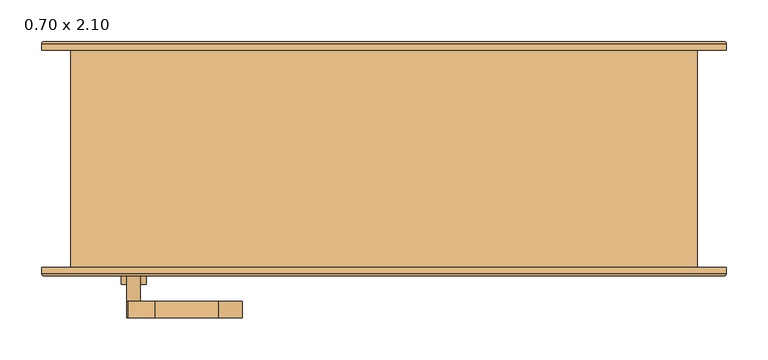
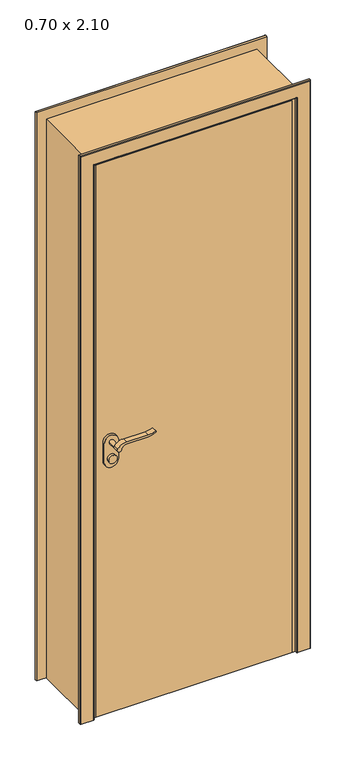
"""IFC4 building model written with IfcOpenShell, lengths in millimetres: door geometry, .CC_ND 300_PORTA SIMPLES DE ABRIR_COM EXTENSÃO : 0.70 x 2.10."""

import ifcopenshell
import ifcopenshell.guid

model = None  # the IFC model being written
_history = None  # IfcOwnerHistory: only IFC2X3 demands one
_inside = {}  # id of a spatial element -> (the spatial element, [elements in it])
_under = {}  # id of a project, library or spatial element -> (it, [spatial elements below it])
_declared = {}  # id of a project -> (the project, [libraries it declares])
_typed = {}  # id of a type object -> (the type object, [elements of that type])
_made_of = {}  # id of a material, layer set ... -> (it, [elements and type objects made of it])


def new_model(schema):
    """Start an empty IFC model of exactly this schema.

    Asked for "IFC4X3", IfcOpenShell would pick the latest addendum, in which some entities
    have other attributes; the version numbers below select the first issue.
    IFC2X3 requires an IfcOwnerHistory on every rooted entity: one is made here for all.
    """
    global model, _history
    if schema == "IFC4X3":
        model = ifcopenshell.file(schema_version=(4, 3, 0, 0))
    else:
        model = ifcopenshell.file(schema=schema)
    _inside.clear()
    _under.clear()
    _declared.clear()
    _typed.clear()
    _made_of.clear()
    _history = None
    if model.schema == "IFC2X3":
        org = make("IfcOrganization", Name="unknown")
        user = make(
            "IfcPersonAndOrganization",
            ThePerson=make("IfcPerson", FamilyName="unknown"),
            TheOrganization=org,
        )
        app = make(
            "IfcApplication",
            ApplicationDeveloper=org,
            Version="unknown",
            ApplicationFullName="unknown",
            ApplicationIdentifier="unknown",
        )
        _history = make(
            "IfcOwnerHistory",
            OwningUser=user,
            OwningApplication=app,
            ChangeAction="ADDED",
            CreationDate=0,
        )
    return model


def make(cls, **values):
    """One entity of the class cls with the attributes given. An attribute that is None is left unset."""
    return model.create_entity(
        cls, **{name: value for name, value in values.items() if value is not None}
    )


def rooted(cls, **values):
    """An entity with a GlobalId (a new one), such as an element, a storey or a relation."""
    return make(cls, GlobalId=ifcopenshell.guid.new(), OwnerHistory=_history, **values)


def si_unit(unit_type, name, prefix=None):
    """IfcSIUnit, for example si_unit("LENGTHUNIT", "METRE", prefix="MILLI")."""
    return make("IfcSIUnit", UnitType=unit_type, Prefix=prefix, Name=name)


def assignment(units):
    """IfcUnitAssignment: the units of a project."""
    return None if units is None else make("IfcUnitAssignment", Units=units)


def point(xyz):
    """IfcCartesianPoint."""
    return None if xyz is None else make("IfcCartesianPoint", Coordinates=xyz)


def direction(xyz):
    """IfcDirection."""
    return None if xyz is None else make("IfcDirection", DirectionRatios=xyz)


def frame(location, z_axis=None, x_axis=None):
    """IfcAxis2Placement3D, a coordinate frame: its origin and axes. An axis left out is left unset."""
    return make(
        "IfcAxis2Placement3D",
        Location=point(location),
        Axis=direction(z_axis),
        RefDirection=direction(x_axis),
    )


def frame_2d(location, x_axis=None):
    """IfcAxis2Placement2D, a coordinate frame in the plane: its origin and x axis."""
    return make(
        "IfcAxis2Placement2D", Location=point(location), RefDirection=direction(x_axis)
    )


def origin():
    """The frame at (0, 0, 0) with its axes left unset."""
    return frame((0.0, 0.0, 0.0))


def origin_with_axes():
    """The frame at (0, 0, 0) with the z axis (0, 0, 1) and the x axis (1, 0, 0) written out."""
    return frame((0.0, 0.0, 0.0), z_axis=(0.0, 0.0, 1.0), x_axis=(1.0, 0.0, 0.0))


def place(relative_to, where):
    """IfcLocalPlacement: puts the frame where relative to a parent placement (None: the world)."""
    return make(
        "IfcLocalPlacement", PlacementRelTo=relative_to, RelativePlacement=where
    )


def context(
    kind, dimensions, precision=None, world=None, true_north=None, identifier=None
):
    """IfcGeometricRepresentationContext, for example the 3D "Model" context."""
    return make(
        "IfcGeometricRepresentationContext",
        ContextIdentifier=identifier,
        ContextType=kind,
        CoordinateSpaceDimension=dimensions,
        Precision=precision,
        WorldCoordinateSystem=world,
        TrueNorth=true_north,
    )


def project(units=None, contexts=None):
    """IfcProject with its units and contexts."""
    return rooted(
        "IfcProject",
        Name="project",
        RepresentationContexts=contexts,
        UnitsInContext=assignment(units),
    )


def spatial(cls, under=None, at=None, **own):
    """A site, building, storey or space (cls), placed at a placement, below another one or the project."""
    s = rooted(cls, ObjectPlacement=at, **own)
    if under is not None:
        _under.setdefault(under.id(), (under, []))[1].append(s)
    return s


def polyline(points):
    """IfcPolyline through the points."""
    return make("IfcPolyline", Points=[point(p) for p in points])


def circle_curve(where, radius):
    """IfcCircle in the frame where."""
    return make("IfcCircle", Position=where, Radius=radius)


def ellipse_curve(where, semi_axis1, semi_axis2):
    """IfcEllipse in the frame where."""
    return make(
        "IfcEllipse", Position=where, SemiAxis1=semi_axis1, SemiAxis2=semi_axis2
    )


def trimmed(basis, trim1, trim2, sense, master):
    """IfcTrimmedCurve: the piece of a basis curve between two trims."""
    return make(
        "IfcTrimmedCurve",
        BasisCurve=basis,
        Trim1=trim1,
        Trim2=trim2,
        SenseAgreement=sense,
        MasterRepresentation=master,
    )


def segment(curve, same_sense, transition):
    """IfcCompositeCurveSegment."""
    return make(
        "IfcCompositeCurveSegment",
        Transition=transition,
        SameSense=same_sense,
        ParentCurve=curve,
    )


def composite_curve(segments, self_intersect=None):
    """IfcCompositeCurve: segments joined end to end."""
    return make("IfcCompositeCurve", Segments=segments, SelfIntersect=self_intersect)


def outline(outer, holes=None, kind="AREA"):
    """IfcArbitraryClosedProfileDef: a profile drawn as a closed curve; with holes, ...WithVoids."""
    if holes is None:
        return make("IfcArbitraryClosedProfileDef", ProfileType=kind, OuterCurve=outer)
    return make(
        "IfcArbitraryProfileDefWithVoids",
        ProfileType=kind,
        OuterCurve=outer,
        InnerCurves=holes,
    )


def extrude(swept, where, along, depth):
    """IfcExtrudedAreaSolid: the profile swept, set in the frame where, extruded along a direction by depth."""
    return make(
        "IfcExtrudedAreaSolid",
        SweptArea=swept,
        Position=where,
        ExtrudedDirection=direction(along),
        Depth=depth,
    )


def faces_of(points, faces, orient=None, outer=None):
    """IfcFace entities. A face is a list of loops; a loop is a list of indices into points, from 0.

    orient and outer hold one flag for each loop. By default every Orientation is true, the
    first loop of a face is its IfcFaceOuterBound and the others are IfcFaceBound.
    """
    made = []
    for i, loops in enumerate(faces):
        bounds = []
        for j, loop in enumerate(loops):
            is_outer = j == 0 if outer is None else outer[i][j]
            bounds.append(
                make(
                    "IfcFaceOuterBound" if is_outer else "IfcFaceBound",
                    Bound=make("IfcPolyLoop", Polygon=[points[k] for k in loop]),
                    Orientation=True if orient is None else orient[i][j],
                )
            )
        made.append(make("IfcFace", Bounds=bounds))
    return made


def faceted_brep(points, faces, orient=None, outer=None, voids=None):
    """IfcFacetedBrep: a solid bounded by flat faces; with voids (closed shells), ...WithVoids."""
    shared = [point(p) for p in points]
    hull = make("IfcClosedShell", CfsFaces=faces_of(shared, faces, orient, outer))
    if voids is None:
        return make("IfcFacetedBrep", Outer=hull)
    return make(
        "IfcFacetedBrepWithVoids",
        Outer=hull,
        Voids=[
            make(cls, CfsFaces=faces_of(shared, fs, o, b)) for cls, fs, o, b in voids
        ],
    )


def shape(context_of_items, identifier, shape_type, items):
    """IfcShapeRepresentation: the items that make up one representation, for example the "Body"."""
    return make(
        "IfcShapeRepresentation",
        ContextOfItems=context_of_items,
        RepresentationIdentifier=identifier,
        RepresentationType=shape_type,
        Items=items,
    )


def source(mapping_origin, context_of_items, identifier, shape_type, items):
    """IfcRepresentationMap: a shape defined once, which mapped items show again and again."""
    return make(
        "IfcRepresentationMap",
        MappingOrigin=mapping_origin,
        MappedRepresentation=shape(context_of_items, identifier, shape_type, items),
    )


def transform(
    local_origin,
    x_axis=None,
    y_axis=None,
    z_axis=None,
    scale=None,
    scale2=None,
    scale3=None,
    uniform=True,
):
    """IfcCartesianTransformationOperator3D, or its non-uniform kind. x_axis, y_axis, z_axis: its Axis1, 2, 3."""
    if uniform:
        return make(
            "IfcCartesianTransformationOperator3D",
            Axis1=direction(x_axis),
            Axis2=direction(y_axis),
            LocalOrigin=point(local_origin),
            Scale=scale,
            Axis3=direction(z_axis),
        )
    return make(
        "IfcCartesianTransformationOperator3DnonUniform",
        Axis1=direction(x_axis),
        Axis2=direction(y_axis),
        LocalOrigin=point(local_origin),
        Scale=scale,
        Axis3=direction(z_axis),
        Scale2=scale2,
        Scale3=scale3,
    )


def mapped(mapping_source, mapping_target):
    """IfcMappedItem: shows the shape of a source again, moved by a transform."""
    return make(
        "IfcMappedItem", MappingSource=mapping_source, MappingTarget=mapping_target
    )


def made_of(thing, what):
    """Note that an element or type object is made of a material, layer set ...; save() writes the relation."""
    if what is not None:
        _made_of.setdefault(what.id(), (what, []))[1].append(thing)
    return thing


def element(
    cls,
    number,
    at=None,
    inside=None,
    cuts=None,
    type_object=None,
    material=None,
    context=None,
    identifier="Body",
    shape_type=None,
    held_by="IfcProductDefinitionShape",
    body=None,
    shapes=None,
    **own,
):
    """One element of the class cls, such as IfcWall. Its Tag is "e" and its number.

    at: its placement. inside: the storey or other place that contains it. cuts: it is an
    opening in that element (IfcRelVoidsElement). A single representation is given by context,
    identifier, shape_type and body (its items); several are given by shapes. held_by: the class
    of the entity that holds the representations. save() writes the other relations.
    """
    e = rooted(cls, Tag="e%d" % number, ObjectPlacement=at, **own)
    if body is not None:
        shapes = [shape(context, identifier, shape_type, body)]
    if shapes is not None:
        e.Representation = make(held_by, Representations=shapes)
    if inside is not None:
        _inside.setdefault(inside.id(), (inside, []))[1].append(e)
    if cuts is not None:
        rooted(
            "IfcRelVoidsElement", RelatingBuildingElement=cuts, RelatedOpeningElement=e
        )
    if type_object is not None:
        _typed.setdefault(type_object.id(), (type_object, []))[1].append(e)
    return made_of(e, material)


def aggregate(whole, parts):
    """IfcRelAggregates: a whole, such as a stair, and the parts it consists of."""
    return rooted("IfcRelAggregates", RelatingObject=whole, RelatedObjects=parts)


def save(model, path):
    """Write the relations noted so far, then the file.

    IfcRelAggregates (storeys below a building ...), IfcRelContainedInSpatialStructure (elements
    in a storey), IfcRelDefinesByType, IfcRelAssociatesMaterial and IfcRelDeclares: one each for
    every whole, place, type object, material and project.
    """
    for whole, parts in _under.values():
        aggregate(whole, parts)
    for where, things in _inside.values():
        rooted(
            "IfcRelContainedInSpatialStructure",
            RelatedElements=things,
            RelatingStructure=where,
        )
    for kind, things in _typed.values():
        rooted("IfcRelDefinesByType", RelatedObjects=things, RelatingType=kind)
    for what, things in _made_of.values():
        rooted("IfcRelAssociatesMaterial", RelatedObjects=things, RelatingMaterial=what)
    for by, libraries in _declared.values():
        rooted("IfcRelDeclares", RelatingContext=by, RelatedDefinitions=libraries)
    model.write(path)


def plane_surface(at):
    """IfcPlane: the flat surface through the origin of the frame at, square to its z axis."""
    return make("IfcPlane", Position=at)


def cylinder_surface(at, radius):
    """IfcCylindricalSurface: all points at the distance radius from the z axis of the frame at."""
    return make("IfcCylindricalSurface", Position=at, Radius=radius)


def advanced_brep(points, edges, surfaces, faces):
    """IfcAdvancedBrep: a solid bounded by faces that lie on surfaces and meet in shared edges.

    An edge is (start, end): straight between two places in points (the first is 0);
    or (start, end, curve); or (start, end, curve, False) where it runs against its curve.
    A face is (place in surfaces, loops), or (place, loops, False) where it looks against
    its surface's normal. A loop lists edges by number (the first is 1), with a minus sign
    where the edge is run from its end to its start. The first loop is the outer one.
    """
    corners = [point(p) for p in points]
    vertices = [make("IfcVertexPoint", VertexGeometry=c) for c in corners]
    made = []
    for start, end, *more in edges:
        made.append(
            make(
                "IfcEdgeCurve",
                EdgeStart=vertices[start],
                EdgeEnd=vertices[end],
                EdgeGeometry=more[0] if more else make("IfcPolyline", Points=[corners[start], corners[end]]),
                SameSense=more[1] if len(more) > 1 else True,
            )
        )
    hull = []
    for where, loops, *sense in faces:
        bounds = []
        for j, loop in enumerate(loops):
            ring = [make("IfcOrientedEdge", EdgeElement=made[abs(k) - 1], Orientation=k > 0) for k in loop]
            bounds.append(
                make(
                    "IfcFaceOuterBound" if j == 0 else "IfcFaceBound",
                    Bound=make("IfcEdgeLoop", EdgeList=ring),
                    Orientation=True,
                )
            )
        hull.append(make("IfcAdvancedFace", Bounds=bounds, FaceSurface=surfaces[where], SameSense=sense[0] if sense else True))
    return make("IfcAdvancedBrep", Outer=make("IfcClosedShell", CfsFaces=hull))


def door_0_70_x_2_10_365ff999(model_context):
    return source(origin(), model_context, "Body", "SolidModel", [
        extrude(outline(composite_curve([segment(trimmed(circle_curve(frame_2d((964.5, -300.0)), 15.0), [point((964.5, -285.0))], [point((964.5, -315.0))], False, "CARTESIAN"), True, "CONTINUOUS"), segment(trimmed(circle_curve(frame_2d((964.5, -300.0)), 15.0), [point((964.5, -315.0))], [point((964.5, -285.0))], False, "CARTESIAN"), True, "CONTINUOUS")], self_intersect=False)), frame((0.0, -163.0, 0.0), z_axis=(0.0, 1.0, 0.0), x_axis=(0.0, 0.0, 1.0)), (0.0, 0.0, 1.0), 10.0),
        extrude(outline(composite_curve([segment(trimmed(circle_curve(frame_2d((964.5, -300.0)), 15.0), [point((964.5, -285.0))], [point((964.5, -315.0))], False, "CARTESIAN"), True, "CONTINUOUS"), segment(trimmed(circle_curve(frame_2d((964.5, -300.0)), 15.0), [point((964.5, -315.0))], [point((964.5, -285.0))], False, "CARTESIAN"), True, "CONTINUOUS")], self_intersect=False)), frame((0.0, -103.0, 0.0), z_axis=(0.0, 1.0, 0.0), x_axis=(0.0, 0.0, 1.0)), (0.0, 0.0, 1.0), 10.0),
        extrude(outline(composite_curve([segment(trimmed(circle_curve(frame_2d((1024.5, -300.0)), 8.0), [point((1029.1523287, -306.5081363))], [point((1024.5, -292.0))], False, "CARTESIAN"), True, "CONTINUOUS"), segment(trimmed(circle_curve(frame_2d((1019.3738613, -274.6138099)), 18.1261387), [point((1024.5, -292.0))], [point((1037.5, -274.6138099))], True, "CARTESIAN"), True, "CONTINUOUS"), segment(polyline([(1037.5, -274.6138099), (1037.5, -198.3564091)]), True, "CONTINUOUS"), segment(trimmed(circle_curve(frame_2d((1096.7709207, -201.9396612)), 59.3791355), [point((1037.5, -198.3564091))], [point((1046.7135558, -170.0))], False, "CARTESIAN"), True, "CONTINUOUS"), segment(polyline([(1046.7135558, -170.0), (1049.5, -170.0)]), True, "CONTINUOUS"), segment(trimmed(circle_curve(frame_2d((1127.7850638, -198.4227909)), 83.2850902), [point((1049.5, -170.0))], [point((1044.5, -198.3564091))], True, "CARTESIAN"), True, "CONTINUOUS"), segment(polyline([(1044.5, -198.3564091), (1044.5, -274.6325667)]), True, "CONTINUOUS"), segment(trimmed(circle_curve(frame_2d((1007.2555521, -276.3324871)), 37.2832219), [point((1044.5, -274.6325667))], [point((1029.1523287, -306.5081363))], False, "CARTESIAN"), True, "CONTINUOUS")], self_intersect=False)), frame((0.0, -203.0, 0.0), z_axis=(0.0, 1.0, 0.0), x_axis=(0.0, 0.0, 1.0)), (0.0, 0.0, 1.0), 20.0),
        extrude(outline(composite_curve([segment(trimmed(circle_curve(frame_2d((1019.3738682, -274.6138122)), 18.1261318), [point((1024.4999903, -292.0))], [point((1037.5, -274.6138122))], True, "CARTESIAN"), True, "CONTINUOUS"), segment(polyline([(1037.5, -274.6138122), (1037.5, -198.3564091)]), True, "CONTINUOUS"), segment(trimmed(circle_curve(frame_2d((1096.7709207, -201.9396612)), 59.3791355), [point((1037.5, -198.3564091))], [point((1046.7135558, -170.0))], False, "CARTESIAN"), True, "CONTINUOUS"), segment(polyline([(1046.7135558, -170.0), (1049.5, -170.0)]), True, "CONTINUOUS"), segment(trimmed(circle_curve(frame_2d((1127.7850638, -198.4227909)), 83.2850902), [point((1049.5, -170.0))], [point((1044.5, -198.3564091))], True, "CARTESIAN"), True, "CONTINUOUS"), segment(polyline([(1044.5, -198.3564091), (1044.5, -274.6325667)]), True, "CONTINUOUS"), segment(trimmed(circle_curve(frame_2d((1007.2555521, -276.3324871)), 37.2832219), [point((1044.5, -274.6325667))], [point((1029.1523287, -306.5081363))], False, "CARTESIAN"), True, "CONTINUOUS"), segment(trimmed(circle_curve(frame_2d((1024.5, -300.0)), 8.0), [point((1029.1523287, -306.5081363))], [point((1024.4999903, -292.0))], False, "CARTESIAN"), True, "CONTINUOUS")], self_intersect=False)), frame((0.0, -73.0, 0.0), z_axis=(0.0, 1.0, 0.0), x_axis=(0.0, 0.0, 1.0)), (0.0, 0.0, 1.0), 20.0),
        extrude(outline(composite_curve([segment(trimmed(circle_curve(frame_2d((1024.5, -300.0)), 8.0), [point((1024.5, -292.0))], [point((1024.5, -308.0))], False, "CARTESIAN"), True, "CONTINUOUS"), segment(trimmed(circle_curve(frame_2d((1024.5, -300.0)), 8.0), [point((1024.5, -308.0))], [point((1024.5, -292.0))], False, "CARTESIAN"), True, "CONTINUOUS")], self_intersect=False)), frame((0.0, -183.0, 0.0), z_axis=(0.0, 1.0, 0.0), x_axis=(0.0, 0.0, 1.0)), (0.0, 0.0, 1.0), 30.0),
        extrude(outline(composite_curve([segment(trimmed(circle_curve(frame_2d((1024.5, -300.0)), 8.0), [point((1024.5, -292.0))], [point((1024.5, -308.0))], False, "CARTESIAN"), True, "CONTINUOUS"), segment(trimmed(circle_curve(frame_2d((1024.5, -300.0)), 8.0), [point((1024.5, -308.0))], [point((1024.5, -292.0))], False, "CARTESIAN"), True, "CONTINUOUS")], self_intersect=False)), frame((0.0, -103.0, 0.0), z_axis=(0.0, 1.0, 0.0), x_axis=(0.0, 0.0, 1.0)), (0.0, 0.0, 1.0), 30.0),
        extrude(outline(composite_curve([segment(trimmed(circle_curve(frame_2d((954.5, -300.0)), 25.0), [point((954.5, -325.0))], [point((954.5, -275.0))], False, "CARTESIAN"), True, "CONTINUOUS"), segment(polyline([(954.5, -275.0), (1024.5, -275.0)]), True, "CONTINUOUS"), segment(trimmed(circle_curve(frame_2d((1024.5, -300.0)), 25.0), [point((1024.5, -275.0))], [point((1024.5, -325.0))], False, "CARTESIAN"), True, "CONTINUOUS"), segment(polyline([(1024.5, -325.0), (954.5, -325.0)]), True, "CONTINUOUS")], self_intersect=False)), frame((0.0, -153.0, 0.0), z_axis=(0.0, 1.0, 0.0), x_axis=(0.0, 0.0, 1.0)), (0.0, 0.0, 1.0), 10.0),
        extrude(outline(composite_curve([segment(trimmed(circle_curve(frame_2d((954.5, -300.0)), 25.0), [point((954.5, -325.0))], [point((954.5, -275.0))], False, "CARTESIAN"), True, "CONTINUOUS"), segment(polyline([(954.5, -275.0), (1024.5, -275.0)]), True, "CONTINUOUS"), segment(trimmed(circle_curve(frame_2d((1024.5, -300.0)), 25.0), [point((1024.5, -275.0))], [point((1024.5, -325.0))], False, "CARTESIAN"), True, "CONTINUOUS"), segment(polyline([(1024.5, -325.0), (954.5, -325.0)]), True, "CONTINUOUS")], self_intersect=False)), frame((0.0, -113.0, 0.0), z_axis=(0.0, 1.0, 0.0), x_axis=(0.0, 0.0, 1.0)), (0.0, 0.0, 1.0), 10.0),
        advanced_brep(
        [(-410.0, -143.0, 0.0), (-360.0, -143.0, 0.0), (-360.0, -150.0, 0.0), (-363.0, -153.0, 0.0), (-407.0, -153.0, 0.0), (-410.0, -150.0, 0.0), (-410.0, -143.0, 2135.0), (410.0, -143.0, 2135.0), (410.0, -143.0, 0.0), (360.0, -143.0, 0.0), (360.0, -143.0, 2085.0), (-360.0, -143.0, 2085.0), (-360.0, -150.0, 2085.0), (-363.0, -153.0, 2088.0), (363.0, -153.0, 2088.0), (363.0, -153.0, 0.0), (407.0, -153.0, 0.0), (407.0, -153.0, 2132.0), (-407.0, -153.0, 2132.0), (-410.0, -150.0, 2135.0), (410.0, -150.0, 2135.0), (410.0, -150.0, 0.0), (360.0, -150.0, 0.0), (360.0, -150.0, 2085.0)],
        [
            (0, 1),
            (1, 2),
            (2, 3, circle_curve(frame((-363.0, -150.0, 0.0), z_axis=(0.0, 0.0, -1.0), x_axis=(1.0, 0.0, 0.0)), 3.0)),
            (3, 4),
            (4, 5, circle_curve(frame((-407.0, -150.0, 0.0), z_axis=(0.0, 0.0, -1.0), x_axis=(1.0, 0.0, 0.0)), 3.0)),
            (5, 0),
            (0, 6),
            (6, 7),
            (7, 8),
            (8, 9),
            (9, 10),
            (10, 11),
            (11, 1),
            (11, 12),
            (12, 2),
            (12, 13, ellipse_curve(frame((-363.0, -150.0, 2088.0), z_axis=(-0.7071067811865475, 0.0, -0.7071067811865475), x_axis=(0.7071067811865474, 0.0, -0.7071067811865476)), 4.2426407, 3.0)),
            (13, 3),
            (13, 14),
            (14, 15),
            (15, 16),
            (16, 17),
            (17, 18),
            (18, 4),
            (18, 19, ellipse_curve(frame((-407.0, -150.0, 2132.0), z_axis=(-0.7071067811865475, 0.0, -0.7071067811865475), x_axis=(0.7071067811865474, 0.0, -0.7071067811865476)), 4.2426407, 3.0)),
            (19, 5),
            (19, 6),
            (7, 20),
            (20, 21),
            (21, 8),
            (21, 16, circle_curve(frame((407.0, -150.0, 0.0), z_axis=(0.0, 0.0, -1.0), x_axis=(-1.0, 0.0, 0.0)), 3.0)),
            (15, 22, circle_curve(frame((363.0, -150.0, 0.0), z_axis=(0.0, 0.0, -1.0), x_axis=(-1.0, 0.0, 0.0)), 3.0)),
            (22, 9),
            (23, 10),
            (22, 23),
            (14, 23, ellipse_curve(frame((363.0, -150.0, 2088.0), z_axis=(0.7071067811865475, 0.0, -0.7071067811865475), x_axis=(0.7071067811865474, 0.0, 0.7071067811865476)), 4.2426407, 3.0)),
            (20, 17, ellipse_curve(frame((407.0, -150.0, 2132.0), z_axis=(0.7071067811865475, 0.0, -0.7071067811865475), x_axis=(0.7071067811865474, 0.0, 0.7071067811865476)), 4.2426407, 3.0)),
            (23, 12),
            (19, 20),
        ],
        [
            plane_surface(frame((-360.0, -143.0, 0.0), z_axis=(0.0, 0.0, -1.0), x_axis=(0.0, 1.0, 0.0))),
            plane_surface(frame((-410.0, -143.0, 0.0), z_axis=(0.0, 1.0, 0.0), x_axis=(0.0, 0.0, 1.0))),
            plane_surface(frame((-360.0, -143.0, 0.0), z_axis=(1.0, 0.0, 0.0), x_axis=(0.0, 0.0, 1.0))),
            cylinder_surface(frame((-363.0, -150.0, 0.0), z_axis=(0.0, 0.0, -1.0), x_axis=(1.0, 0.0, 0.0)), 3.0),
            plane_surface(frame((-363.0, -153.0, 0.0), z_axis=(0.0, -1.0, 0.0), x_axis=(0.0, 0.0, 1.0))),
            cylinder_surface(frame((-407.0, -150.0, 0.0), z_axis=(0.0, 0.0, -1.0), x_axis=(1.0, 0.0, 0.0)), 3.0),
            plane_surface(frame((-410.0, -150.0, 0.0), z_axis=(-1.0, 0.0, 0.0), x_axis=(0.0, 0.0, 1.0))),
            plane_surface(frame((410.0, -150.0, 2135.0), z_axis=(1.0, 0.0, 0.0), x_axis=(0.0, 0.0, -1.0))),
            plane_surface(frame((360.0, -143.0, 0.0), z_axis=(0.0, 0.0, -1.0), x_axis=(0.0, 1.0, 0.0))),
            plane_surface(frame((360.0, -143.0, 2085.0), z_axis=(-1.0, 0.0, 0.0), x_axis=(0.0, 0.0, -1.0))),
            cylinder_surface(frame((363.0, -150.0, 2085.0), z_axis=(0.0, 0.0, 1.0), x_axis=(-1.0, 0.0, 0.0)), 3.0),
            cylinder_surface(frame((407.0, -150.0, 2085.0), z_axis=(0.0, 0.0, 1.0), x_axis=(-1.0, 0.0, 0.0)), 3.0),
            plane_surface(frame((-360.0, -143.0, 2085.0), z_axis=(0.0, 0.0, -1.0), x_axis=(1.0, 0.0, 0.0))),
            plane_surface(frame((-410.0, -150.0, 2135.0), z_axis=(0.0, 0.0, 1.0), x_axis=(1.0, 0.0, 0.0))),
            cylinder_surface(frame((-360.0, -150.0, 2088.0), z_axis=(-1.0, 0.0, 0.0), x_axis=(0.0, 0.0, -1.0)), 3.0),
            cylinder_surface(frame((-360.0, -150.0, 2132.0), z_axis=(-1.0, 0.0, 0.0), x_axis=(0.0, 0.0, -1.0)), 3.0),
        ],
        [
            (0, [[1, 2, 3, 4, 5, 6]]),
            (1, [[-1, 7, 8, 9, 10, 11, 12, 13]]),
            (2, [[-2, -13, 14, 15]]),
            (3, [[-3, -15, 16, 17]]),
            (4, [[-4, -17, 18, 19, 20, 21, 22, 23]]),
            (5, [[-5, -23, 24, 25]]),
            (6, [[-6, -25, 26, -7]]),
            (7, [[27, 28, 29, -9]]),
            (8, [[-29, 30, -20, 31, 32, -10]]),
            (9, [[33, -11, -32, 34]]),
            (10, [[35, -34, -31, -19]]),
            (11, [[36, -21, -30, -28]]),
            (12, [[-14, -12, -33, 37]]),
            (13, [[-26, 38, -27, -8]]),
            (14, [[-16, -37, -35, -18]]),
            (15, [[-24, -22, -36, -38]]),
        ],
    ),
        advanced_brep(
        [(410.0, 118.0, 0.0), (360.0, 118.0, 0.0), (360.0, 125.0157283, 0.0), (362.9842717, 128.0, 0.0), (407.0342217, 128.0, 0.0), (410.0, 125.0342217, 0.0), (410.0, 118.0, 2135.0), (-410.0, 118.0, 2135.0), (-410.0, 118.0, 0.0), (-360.0, 118.0, 0.0), (-360.0, 118.0, 2085.0), (360.0, 118.0, 2085.0), (360.0, 125.0157283, 2085.0), (362.9842717, 128.0, 2087.9842717), (-362.9842717, 128.0, 2087.9842717), (-362.9842717, 128.0, 0.0), (-407.0342217, 128.0, 0.0), (-407.0342217, 128.0, 2132.0342217), (407.0342217, 128.0, 2132.0342217), (410.0, 125.0342217, 2135.0), (-410.0, 125.0342217, 2135.0), (-410.0, 125.0342217, 0.0), (-360.0, 125.0157283, 0.0), (-360.0, 125.0157283, 2085.0)],
        [
            (0, 1),
            (1, 2),
            (2, 3, circle_curve(frame((362.9842717, 125.0157283, 0.0), z_axis=(0.0, 0.0, -1.0), x_axis=(1.0, 0.0, 0.0)), 2.9842717)),
            (3, 4),
            (4, 5, circle_curve(frame((407.0342217, 125.0342217, 0.0), z_axis=(0.0, 0.0, -1.0), x_axis=(1.0, 0.0, 0.0)), 2.9657783)),
            (5, 0),
            (0, 6),
            (6, 7),
            (7, 8),
            (8, 9),
            (9, 10),
            (10, 11),
            (11, 1),
            (11, 12),
            (12, 2),
            (12, 13, ellipse_curve(frame((362.9842717, 125.0157283, 2087.9842717), z_axis=(0.7071067811865475, 0.0, -0.7071067811865475), x_axis=(-0.7071067811865474, 0.0, -0.7071067811865476)), 4.2203975, 2.9842717)),
            (13, 3),
            (13, 14),
            (14, 15),
            (15, 16),
            (16, 17),
            (17, 18),
            (18, 4),
            (18, 19, ellipse_curve(frame((407.0342217, 125.0342217, 2132.0342217), z_axis=(0.7071067811865475, 0.0, -0.7071067811865475), x_axis=(-0.7071067811865474, 0.0, -0.7071067811865476)), 4.1942438, 2.9657783)),
            (19, 5),
            (19, 6),
            (7, 20),
            (20, 21),
            (21, 8),
            (21, 16, circle_curve(frame((-407.0342217, 125.0342217, 0.0), z_axis=(0.0, 0.0, -1.0), x_axis=(-1.0, 0.0, 0.0)), 2.9657783)),
            (15, 22, circle_curve(frame((-362.9842717, 125.0157283, 0.0), z_axis=(0.0, 0.0, -1.0), x_axis=(-1.0, 0.0, 0.0)), 2.9842717)),
            (22, 9),
            (23, 10),
            (22, 23),
            (14, 23, ellipse_curve(frame((-362.9842717, 125.0157283, 2087.9842717), z_axis=(-0.7071067811865475, 0.0, -0.7071067811865475), x_axis=(-0.7071067811865474, 0.0, 0.7071067811865476)), 4.2203975, 2.9842717)),
            (20, 17, ellipse_curve(frame((-407.0342217, 125.0342217, 2132.0342217), z_axis=(-0.7071067811865475, 0.0, -0.7071067811865475), x_axis=(-0.7071067811865474, 0.0, 0.7071067811865476)), 4.1942438, 2.9657783)),
            (23, 12),
            (19, 20),
        ],
        [
            plane_surface(frame((360.0, 118.0, 0.0), z_axis=(0.0, 0.0, -1.0), x_axis=(0.0, 1.0, 0.0))),
            plane_surface(frame((410.0, 118.0, 0.0), z_axis=(0.0, -1.0, 0.0), x_axis=(0.0, 0.0, 1.0))),
            plane_surface(frame((360.0, 118.0, 0.0), z_axis=(-1.0, 0.0, 0.0), x_axis=(0.0, 0.0, 1.0))),
            cylinder_surface(frame((362.9842717, 125.0157283, 0.0), z_axis=(0.0, 0.0, -1.0), x_axis=(1.0, 0.0, 0.0)), 2.9842717),
            plane_surface(frame((362.9842717, 128.0, 0.0), z_axis=(0.0, 1.0, 0.0), x_axis=(0.0, 0.0, 1.0))),
            cylinder_surface(frame((407.0342217, 125.0342217, 0.0), z_axis=(0.0, 0.0, -1.0), x_axis=(1.0, 0.0, 0.0)), 2.9657783),
            plane_surface(frame((410.0, 125.0342217, 0.0), z_axis=(1.0, 0.0, 0.0), x_axis=(0.0, 0.0, 1.0))),
            plane_surface(frame((-410.0, 125.0342217, 2135.0), z_axis=(-1.0, 0.0, 0.0), x_axis=(0.0, 0.0, -1.0))),
            plane_surface(frame((-360.0, 118.0, 0.0), z_axis=(0.0, 0.0, -1.0), x_axis=(0.0, 1.0, 0.0))),
            plane_surface(frame((-360.0, 118.0, 2085.0), z_axis=(1.0, 0.0, 0.0), x_axis=(0.0, 0.0, -1.0))),
            cylinder_surface(frame((-362.9842717, 125.0157283, 2085.0), z_axis=(0.0, 0.0, 1.0), x_axis=(-1.0, 0.0, 0.0)), 2.9842717),
            cylinder_surface(frame((-407.0342217, 125.0342217, 2085.0), z_axis=(0.0, 0.0, 1.0), x_axis=(-1.0, 0.0, 0.0)), 2.9657783),
            plane_surface(frame((360.0, 118.0, 2085.0), z_axis=(0.0, 0.0, -1.0), x_axis=(-1.0, 0.0, 0.0))),
            plane_surface(frame((410.0, 125.0342217, 2135.0), z_axis=(0.0, 0.0, 1.0), x_axis=(-1.0, 0.0, 0.0))),
            cylinder_surface(frame((360.0, 125.0157283, 2087.9842717), z_axis=(1.0, 0.0, 0.0), x_axis=(0.0, 0.0, 1.0)), 2.9842717),
            cylinder_surface(frame((360.0, 125.0342217, 2132.0342217), z_axis=(1.0, 0.0, 0.0), x_axis=(0.0, 0.0, 1.0)), 2.9657783),
        ],
        [
            (0, [[1, 2, 3, 4, 5, 6]]),
            (1, [[-1, 7, 8, 9, 10, 11, 12, 13]]),
            (2, [[-2, -13, 14, 15]]),
            (3, [[-3, -15, 16, 17]]),
            (4, [[-4, -17, 18, 19, 20, 21, 22, 23]]),
            (5, [[-5, -23, 24, 25]]),
            (6, [[-6, -25, 26, -7]]),
            (7, [[27, 28, 29, -9]]),
            (8, [[-29, 30, -20, 31, 32, -10]]),
            (9, [[33, -11, -32, 34]]),
            (10, [[35, -34, -31, -19]]),
            (11, [[36, -21, -30, -28]]),
            (12, [[-14, -12, -33, 37]]),
            (13, [[-26, 38, -27, -8]]),
            (14, [[-16, -37, -35, -18]]),
            (15, [[-24, -22, -36, -38]]),
        ],
    ),
        faceted_brep([(342.0, 118.0, 0.0), (375.0, 118.0, 0.0), (375.0, -143.0, 0.0), (350.0, -143.0, 0.0), (350.0, -113.0, 0.0), (342.0, -113.0, 0.0), (342.0, 118.0, 2067.0), (-342.0, 118.0, 2067.0), (-342.0, 118.0, 0.0), (-375.0, 118.0, 0.0), (-375.0, 118.0, 2100.0), (375.0, 118.0, 2100.0), (375.0, -143.0, 2100.0), (-375.0, -143.0, 2100.0), (-375.0, -143.0, 0.0), (-350.0, -143.0, 0.0), (-350.0, -143.0, 2075.0), (350.0, -143.0, 2075.0), (350.0, -113.0, 2075.0), (-350.0, -113.0, 2075.0), (-350.0, -113.0, 0.0), (-342.0, -113.0, 0.0), (-342.0, -113.0, 2067.0), (342.0, -113.0, 2067.0)], [[[0, 1, 2, 3, 4, 5]], [[1, 0, 6, 7, 8, 9, 10, 11]], [[2, 1, 11, 12]], [[3, 2, 12, 13, 14, 15, 16, 17]], [[4, 3, 17, 18]], [[5, 4, 18, 19, 20, 21, 22, 23]], [[0, 5, 23, 6]], [[7, 22, 21, 8]], [[8, 21, 20, 15, 14, 9]], [[13, 10, 9, 14]], [[19, 16, 15, 20]], [[12, 11, 10, 13]], [[18, 17, 16, 19]], [[6, 23, 22, 7]]]),
        extrude(outline(polyline([(-350.0, -113.0), (350.0, -113.0), (350.0, -143.0), (-350.0, -143.0), (-350.0, -113.0)])), origin_with_axes(), (0.0, 0.0, 1.0), 2075.0),
    ])


if __name__ == "__main__":
    model = new_model("IFC4")
    model_context = context("Model", 3, world=origin())
    ifc_project = project(units=[si_unit("LENGTHUNIT", "METRE", prefix="MILLI")], contexts=[model_context])
    site = spatial("IfcSite", under=ifc_project)
    building = spatial("IfcBuilding", under=site)
    placement = place(None, origin())
    door_0_70_x_2_10_shape = door_0_70_x_2_10_365ff999(model_context)
    element("IfcDoor", 1, ObjectType=".CC_ND 300_PORTA SIMPLES DE ABRIR_COM EXTENSÃO : 0.70 x 2.10", at=placement, inside=building, context=model_context, shape_type="MappedRepresentation", body=[
        mapped(door_0_70_x_2_10_shape, transform((0.0, 0.0, 0.0), x_axis=(1.0, 0.0, 0.0), y_axis=(0.0, 1.0, 0.0), z_axis=(0.0, 0.0, 1.0))),
    ])
    save(model, "model.ifc")

# Revit data of these elements
# Type ".CC_ND 300_PORTA SIMPLES DE ABRIR_COM EXTENSÃO : 0.70 x 2.10"
#   Type Mark = "155"
#   Rough Width = 0.75 m
#   Espessura moldura externa = 0.01 m
#   Espessura moldura interna = 0.01 m
#   Largura moldura = 0.05 m
#   Extensão acabamento exterior [instance default] = 0.00 m
#   Extensão acabamento interior [instance default] = 0.00 m
#   Espessura batente = 0.025 m
#   Thickness = 0.03 m
#   Altura batente = 2.085 m
#   Aux Arco [instance default] = 0.70 m
#   Rough Height = 2.125 m
#   Height = 2.10 m
#   Width = 0.70 m
#   Moldura interna [instance default] = yes
#   Moldura externa [instance default] = yes
#   Porta = .MADEIRA COM PINTURA ESMALTE BRANCO ACETINADO
#   Moldura = .MADEIRA COM PINTURA ESMALTE BRANCO ACETINADO
#   Maçaneta = .ALUMÍNIO
#   Batente = .MADEIRA COM PINTURA ESMALTE BRANCO ACETINADO
#   Function = (empty or 0)
#   Wall Closure = (empty or 0)
# Element 1 (IfcDoor, ".CC_ND 300_PORTA SIMPLES DE ABRIR_COM EXTENSÃO : 0.70 x 2.10")
#   Extensão acabamento interior = 0.025 m
#   Aux Arco = 0.725 m
#   Materials on its faces: ".MADEIRA COM PINTURA ESMALTE BRANCO ACETINADO", ".ALUMÍNIO"
# Materials
#   ".MADEIRA COM PINTURA ESMALTE BRANCO ACETINADO": class ".CC_MADEIRAS", colour RGB 240 240 240, transparency 0, Description = "Madeira com pintura esmalte branco acetinado.", Cost = 0
#   ".ALUMÍNIO": class "CC_METAIS", colour RGB 244 244 244, transparency 0, Description = "Material alumínio", Cost = 0
